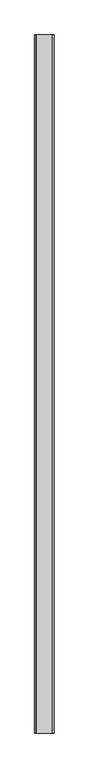
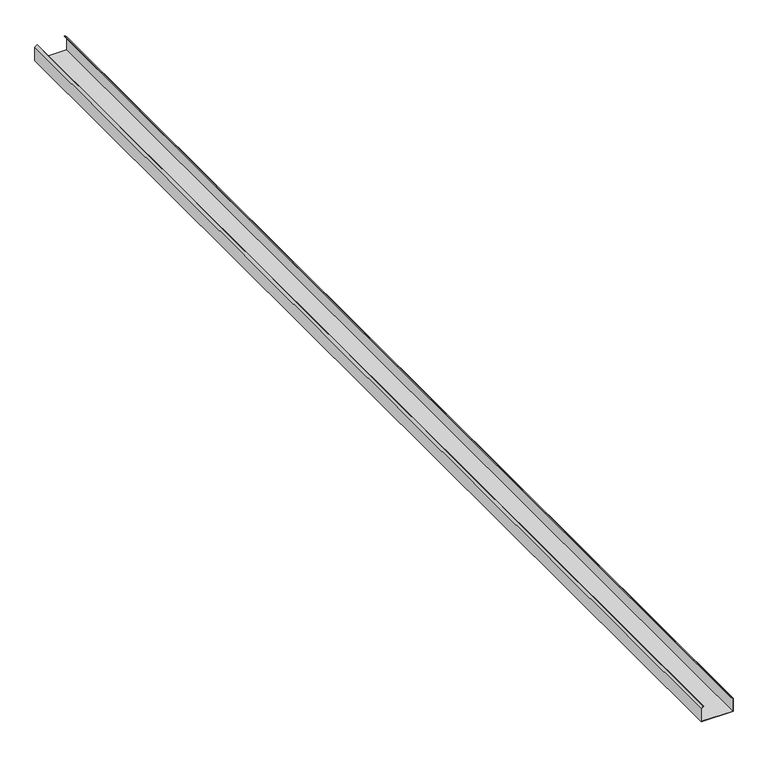
"""IFC4 building model written with IfcOpenShell, lengths in millimetres: proxy geometry, Generic Models 7:Generic Models 1:1:Generic Models 1:1 : Generic Models 7:Generic Models 1:337419:49 : Generic Models 7:Generic Models 1:1:Generic Models 1:1 : Generic Models 7:Generic Models 1:337419:306201."""

from ifc_helpers import new_model, si_unit, frame, origin, place, context, project, spatial, polyline, outline, extrude, source, transform, mapped, element, save


def generic_models_69d90831(model_context):
    return source(origin(), model_context, "Body", "SweptSolid", [
        extrude(outline(polyline([(3617.9125, 560568.8617239), (3706.8125, 560568.8617239), (3719.057604, 560554.2685773), (3716.9294367, 560552.482833), (3705.517039, 560566.0835989), (3620.690625, 560566.0835989), (3620.690625, 560368.4398489), (3705.517039, 560368.4398489), (3716.9294367, 560382.0406149), (3719.057604, 560380.2548706), (3706.8125, 560365.6617239), (3617.9125, 560365.6617239), (3617.9125, 560568.8617239)])), frame((0.0, -550498.7163841, 0.0), z_axis=(0.0, 1.0, 0.0), x_axis=(0.0, 0.0, 1.0)), (0.0, 0.0, 1.0), 7315.2),
    ])


if __name__ == "__main__":
    model = new_model("IFC4")
    model_context = context("Model", 3, world=origin())
    ifc_project = project(units=[si_unit("LENGTHUNIT", "METRE", prefix="MILLI")], contexts=[model_context])
    site = spatial("IfcSite", under=ifc_project)
    building = spatial("IfcBuilding", under=site)
    placement = place(None, origin())
    generic_models_shape = generic_models_69d90831(model_context)
    element("IfcBuildingElementProxy", 1, Name="Generic Models 7:Generic Models 1:1:Generic Models 1:1 : Generic Models 7:Generic Models 1:337419:49 : Generic Models 7:Generic Models 1:1:Generic Models 1:1 : Generic Models 7:Generic Models 1:337419:306201", ObjectType="Generic Models 7:Generic Models 1:1:Generic Models 1:1 : Generic Models 7:Generic Models 1:337419:49 : Generic Models 7:Generic Models 1:1:Generic Models 1:1 : Generic Models 7:Generic Models 1:337419:306201", at=placement, inside=building, context=model_context, shape_type="MappedRepresentation", body=[
        mapped(generic_models_shape, transform((0.0, 0.0, 0.0), x_axis=(1.0, 0.0, 0.0), y_axis=(0.0, 1.0, 0.0), z_axis=(0.0, 0.0, 1.0))),
    ])
    save(model, "model.ifc")

# Revit data of these elements
# Type "Generic Models 7:Generic Models 1:1:Generic Models 1:1 : Generic Models 7:Generic Models 1:337419:49 : Generic Models 7:Generic Models 1:1:Generic Models 1:1 : Generic Models 7:Generic Models 1:337419:306201"
#   NameOverride = "Generic Models 7:Generic Models 1:1:Generic Models 1:1 : Generic Models 7:Generic Models 1:337419:306201"
#   ObjectTypeOverride = "Generic Models 1:1 : Generic Models 7:Generic Models 1:337419"
#   Reference = "Generic Models 1"
#   Tag = "306201"
# Element 1 (IfcBuildingElementProxy, "Generic Models 7:Generic Models 1:1:Generic Models 1:1 : Generic Models 7:Generic Models 1:337419:49 : Generic Models 7:Generic Models 1:1:Generic Models 1:1 : Generic Models 7:Generic Models 1:337419:306201")
#   Materials on its faces: "CEE' SECTION (8.0x3.5C - SEE STRUCT. DWGS)"
# Materials
#   "CEE' SECTION (8.0x3.5C - SEE STRUCT. DWGS)": class "Unassigned", colour RGB 210 209 208, transparency 0, Keynote = "M05121300.02", Cost = 0
